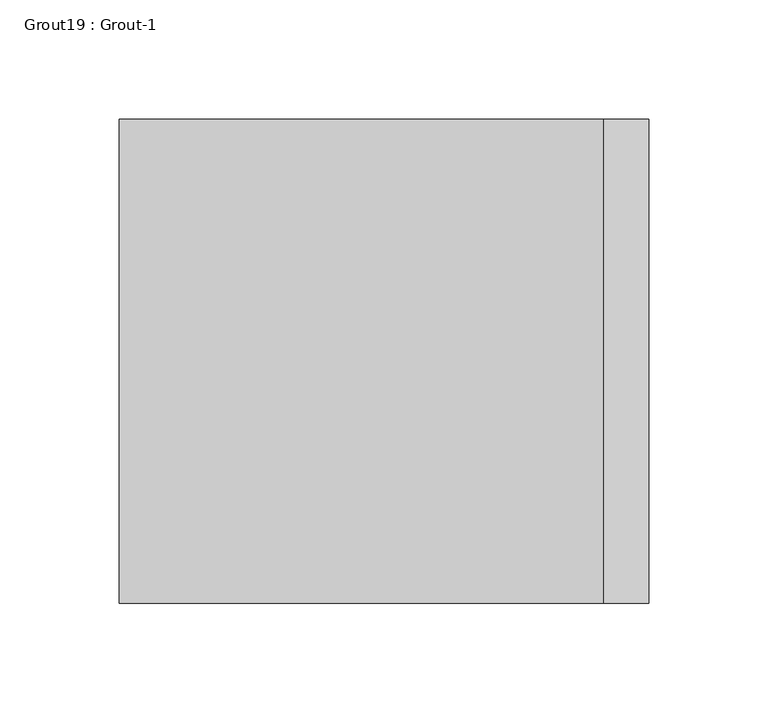
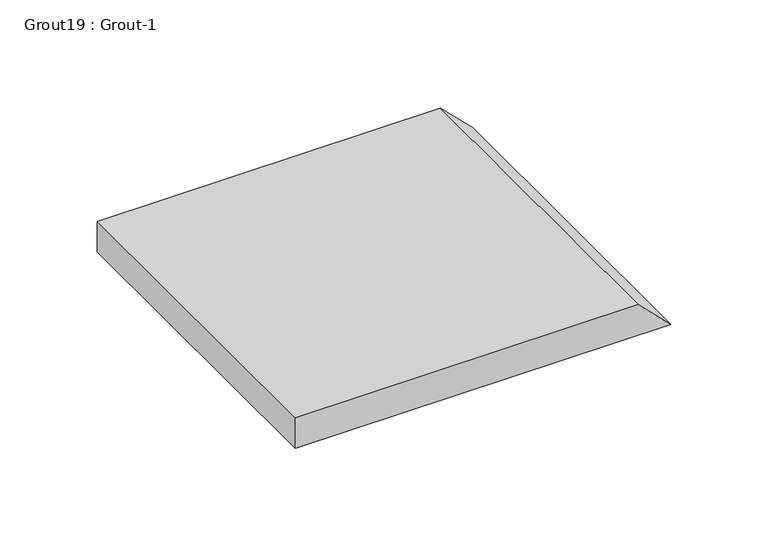
"""IFC4 building model written with IfcOpenShell, lengths in millimetres: proxy geometry, Grout19 : Grout-1."""

from ifc_helpers import new_model, si_unit, frame, origin, place, context, project, spatial, polyline, outline, extrude, source, transform, mapped, element, save


def grout19_grout_1_13d29c56(model_context):
    return source(origin(), model_context, "Body", "SweptSolid", [
        extrude(outline(polyline([(19.05, 587569.0934739), (19.05, 587365.8934739), (0.0, 587365.8934739), (0.0, 587588.1434739), (19.05, 587569.0934739)])), frame((0.0, -536468.3913841, 0.0), z_axis=(0.0, 1.0, 0.0), x_axis=(0.0, 0.0, 1.0)), (0.0, 0.0, 1.0), 203.2),
    ])


if __name__ == "__main__":
    model = new_model("IFC4")
    model_context = context("Model", 3, world=origin())
    ifc_project = project(units=[si_unit("LENGTHUNIT", "METRE", prefix="MILLI")], contexts=[model_context])
    site = spatial("IfcSite", under=ifc_project)
    building = spatial("IfcBuilding", under=site)
    placement = place(None, origin())
    grout19_grout_1_shape = grout19_grout_1_13d29c56(model_context)
    element("IfcBuildingElementProxy", 1, Name="Grout19 : Grout-1", ObjectType="Grout19 : Grout-1", at=placement, inside=building, context=model_context, shape_type="MappedRepresentation", body=[
        mapped(grout19_grout_1_shape, transform((0.0, 0.0, 0.0), x_axis=(1.0, 0.0, 0.0), y_axis=(0.0, 1.0, 0.0), z_axis=(0.0, 0.0, 1.0))),
    ])
    save(model, "model.ifc")

# Revit data of these elements
# Element 1 (IfcBuildingElementProxy, "Grout19 : Grout-1")
#   Materials on its faces: "3/4\" NON SHRINK GROUT"
# Materials
#   "3/4\" NON SHRINK GROUT": class "Generic", colour RGB 145 145 143, transparency 0, Cost = 0
